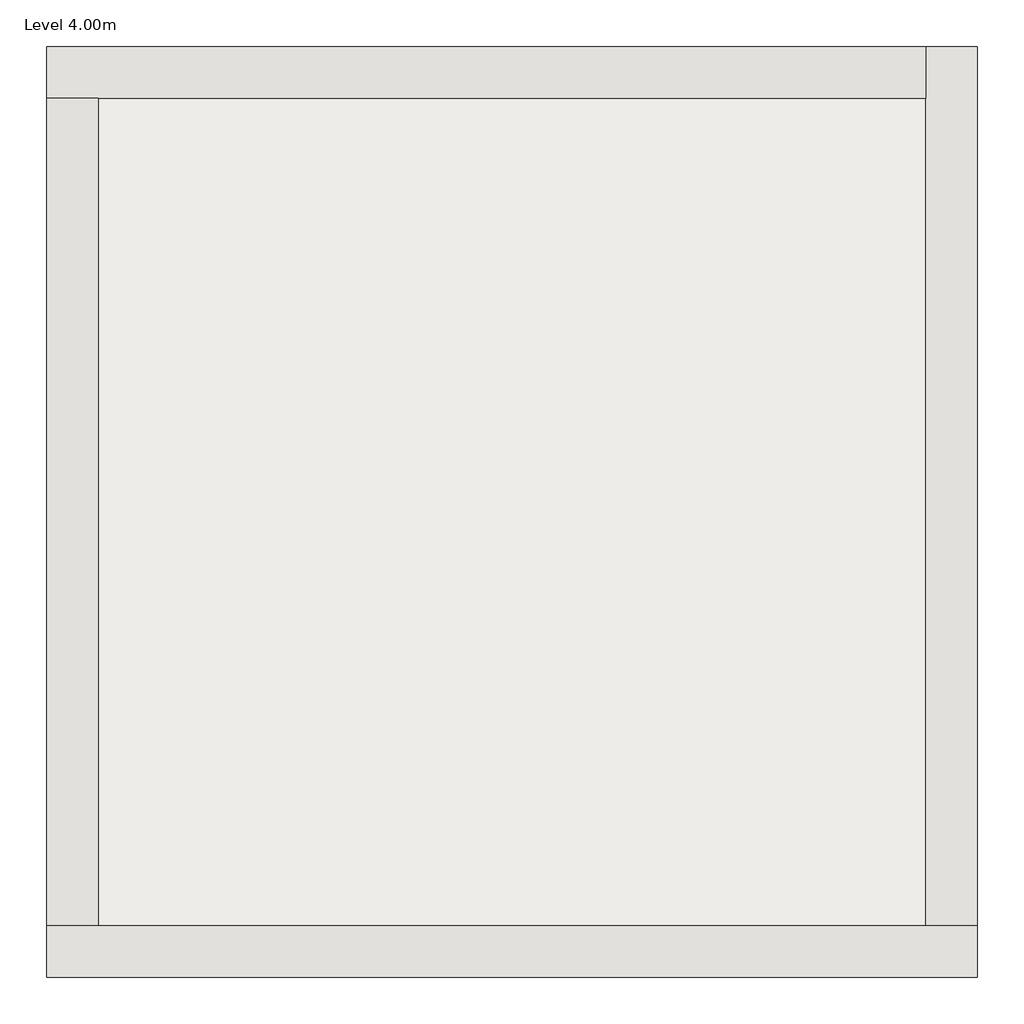
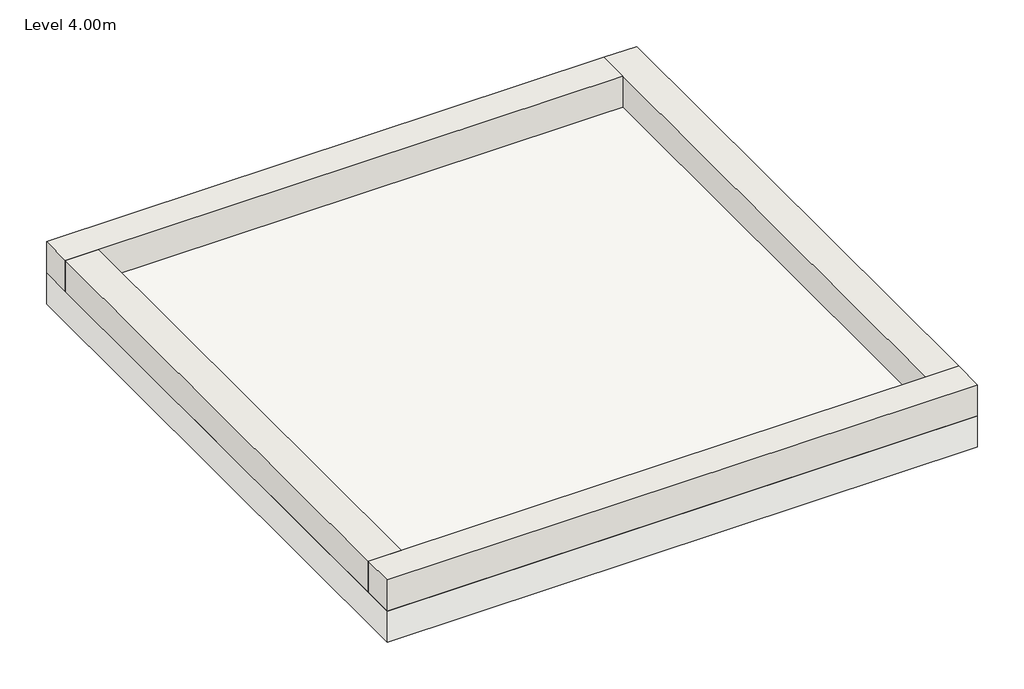
# One storey: 4 walls, 1 slab.
"""IFC4 building model written with IfcOpenShell, lengths in millimetres."""

from ifc_helpers import new_model, si_unit, frame, origin, place, context, project, spatial, polyline, outline, extrude, faceted_brep, element, save

model = new_model("IFC4")

# Units and contexts
model_context = context("Model", 3, world=origin())
ifc_project = project(units=[si_unit("LENGTHUNIT", "METRE", prefix="MILLI")], contexts=[model_context])

# Site, building, storey
site = spatial("IfcSite", under=ifc_project)
building = spatial("IfcBuilding", under=site)
storey = spatial("IfcBuildingStorey", under=building, Name="Level 4.00m", Elevation=4000.0)

# Slab
placement = place(None, origin())
element("IfcSlab", 1, ObjectType="FOR INT AC-NH", at=placement, inside=storey, context=model_context, shape_type="SweptSolid", body=[
    extrude(outline(polyline([(9000.0000251, -1000.0058651), (0.0, -1000.0058651), (0.0, 7999.99416), (9000.0000251, 7999.99416), (9000.0000251, -1000.0058651)])), frame((0.0, 0.0, 3500.0000028), z_axis=(0.0, 0.0, 1.0), x_axis=(1.0, 0.0, 0.0)), (0.0, 0.0, 1.0), 499.9999972),
])

# Walls
element("IfcWall", 2, ObjectType="MURO EXTERIOR0.60", at=placement, inside=storey, context=model_context, shape_type="Brep", body=[
    faceted_brep([(0.0, -1000.0058651, 4000.0), (9000.000032, -1000.0058651, 4000.0), (9000.000032, -1000.0058651, 4499.99392), (0.0, -1000.0058651, 4499.99392), (0.0, -500.0058491, 4000.0), (0.0, -500.0058491, 4499.99392), (500.000016, -500.0058491, 4499.99392), (8500.000016, -500.0058491, 4499.99392), (9000.000032, -500.0058491, 4499.99392), (9000.000032, -500.0058491, 4000.0), (8500.000016, -500.0058491, 4000.0), (500.000016, -500.0058491, 4000.0)], [[[0, 1, 2, 3]], [[4, 5, 6, 7, 8, 9, 10, 11]], [[1, 0, 4, 11, 10, 9]], [[3, 2, 8, 7, 6, 5]], [[2, 1, 9, 8]], [[0, 3, 5, 4]]]),
])
element("IfcWall", 3, ObjectType="MURO EXTERIOR0.60", at=placement, inside=storey, context=model_context, shape_type="Brep", body=[
    faceted_brep([(9000.000032, -500.0058491, 4000.0), (9000.000032, 7999.99416, 4000.0), (9000.000032, 7999.99416, 4499.99392), (9000.000032, -500.0058491, 4499.99392), (8500.000016, -500.0058491, 4000.0), (8500.000016, -500.0058491, 4499.99392), (8500.000016, 7499.994144, 4499.99392), (8500.000016, 7999.99416, 4499.99392), (8500.000016, 7999.99416, 4000.0), (8500.000016, 7499.994144, 4000.0)], [[[0, 1, 2, 3]], [[4, 5, 6, 7, 8, 9]], [[1, 0, 4, 9, 8]], [[3, 2, 7, 6, 5]], [[2, 1, 8, 7]], [[0, 3, 5, 4]]]),
])
element("IfcWall", 4, ObjectType="MURO EXTERIOR0.60", at=placement, inside=storey, context=model_context, shape_type="Brep", body=[
    faceted_brep([(8500.000016, 7999.99416, 4000.0), (0.0, 7999.99416, 4000.0), (0.0, 7999.99416, 4499.99392), (8500.000016, 7999.99416, 4499.99392), (8500.000016, 7499.994144, 4000.0), (8500.000016, 7499.994144, 4499.99392), (500.000016, 7499.994144, 4499.99392), (0.0, 7499.994144, 4499.99392), (0.0, 7499.994144, 4000.0), (500.000016, 7499.994144, 4000.0)], [[[0, 1, 2, 3]], [[4, 5, 6, 7, 8, 9]], [[1, 0, 4, 9, 8]], [[3, 2, 7, 6, 5]], [[2, 1, 8, 7]], [[0, 3, 5, 4]]]),
])
element("IfcWall", 5, ObjectType="MURO EXTERIOR0.60", at=placement, inside=storey, context=model_context, shape_type="SweptSolid", body=[
    extrude(outline(polyline([(0.0, -500.0058491), (0.0, 7499.994144), (500.000016, 7499.994144), (500.000016, -500.0058491), (0.0, -500.0058491)])), frame((0.0, 0.0, 4000.0), z_axis=(0.0, 0.0, 1.0), x_axis=(1.0, 0.0, 0.0)), (0.0, 0.0, 1.0), 499.99392),
])

save(model, "model.ifc")

# Revit data of these elements
# Type "FOR INT AC-NH"
#   Type Comments = "CTE"
#   Description = "Concrete Floor, 100mm thick, Interior Function"
#   Assembly Code = "B1010"
#   Type Mark = "AF01"
#   Function = 0
#   Layers, outside or top first: 0.010 m "Plaqueta o baldosa de gres" (function 4); 0.055 m "Mortero de cemento o cal para albañilería y para revoco-enlucido d entre 1000 y 1250" (function 4); 0.120 m "Poliestireno Expandido XPS" (function 4); 0.250 m "FU Entrevigado cerámico -Canto 250 mm" (function 1); 0.050 m "Cámara de aire sin ventilar horizontal 5 cm" (function 5); 0.015 m "Placa de yeso laminado (PYL) d entre 750 y 900" (function 5)
# Type "MURO EXTERIOR0.60"
#   Description = "Metal Studs with Brick over sheathing on exterior and Gypsum Wall Board (GWB) on interior, Exterior Function"
#   Assembly Code = "B2010158"
#   Type Mark = "W-02"
#   Layers, outside or top first: 0.030 m no material (function 1); 0.140 m no material (function 1); 0.240 m no material (function 1); 0.010 m no material (function 1); 0.050 m no material (function 1); 0.015 m no material (function 1); 0.015 m no material (function 1)
# Element 1 (IfcSlab, "FOR INT AC-NH")
#   Height Offset From Level = 0.000 m
#   Phase Created = New Construction
#   Materials on its faces: "Placa de yeso laminado (PYL) d entre 750 y 900", "Plaqueta o baldosa de gres"
# Elements 2, 3, 4, 5 (IfcWall, "MURO EXTERIOR0.60")
#   Top Offset = 0.000 m
#   Base Offset = 0.000 m
#   Unconnected Height = 0.499994 m
#   wall height = 0.499994 m
#   Phase Created = New Construction
#   Base Constraint = Level 4.00m
#   Materials on its faces: "Default Wall"
# Materials
#   "Plaqueta o baldosa de gres": class "Cerámicos", colour RGB 0 0 0, transparency 0, Model = "2.29999995232", Comments = "Cp: 1000 J/kgK", Description = "HULC Import | Density: 2500 kg/m3"
#   "Mortero de cemento o cal para albañilería y para revoco-enlucido d entre 1000 y 1250": class "Morteros", colour RGB 0 0 0, transparency 0, Comments = "CTE"
#   "Poliestireno Expandido XPS": class "Plásticos", colour RGB 0 0 0, transparency 0, Model = "0.0340000018477", Comments = "Cp: 800 J/kgK", Description = "HULC Import | Density: 1500 kg/m3"
#   "FU Entrevigado cerámico -Canto 250 mm": class "Forjados unidireccionales", colour RGB 0 0 0, transparency 0, Comments = "CTE"
#   "Cámara de aire sin ventilar horizontal 5 cm": class "Cámaras de aire", colour RGB 0 0 0, transparency 0, Comments = "CTE"
#   "Placa de yeso laminado (PYL) d entre 750 y 900": class "Yesos", colour RGB 0 0 0, transparency 0, Model = "0.25", Comments = "Cp: 1000 J/kgK", Description = "HULC Import | Density: 825 kg/m3"
#   "Default Wall": class "Miscellaneous", colour RGB 192 192 192, transparency 0, Cost = 0
